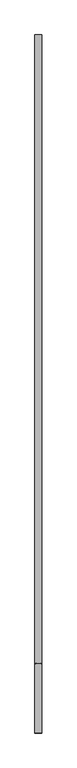
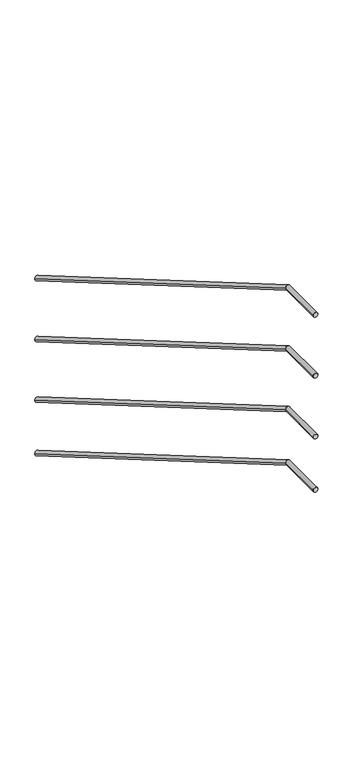
"""IFC4 building model written with IfcOpenShell, lengths in millimetres: railing geometry."""

from ifc_helpers import new_model, si_unit, frame, origin, place, context, project, spatial, circle_curve, ellipse_curve, source, transform, mapped, element, save
from ifc_brep_helpers import plane_surface, cylinder_surface, advanced_brep


def railing_4ce2e709(model_context):
    return source(origin(), model_context, "Body", "AdvancedBrep", [
        advanced_brep(
        [(-340.4, 15799.5208589, 8657.5963084), (-310.4, 15799.5208589, 8657.5963084), (-340.4, 13095.4656218, 10234.9618634), (-310.4, 13095.4656218, 10234.9618634), (-340.4, 12799.5208589, 10234.9618634), (-310.4, 12799.5208589, 10234.9618634)],
        [
            (0, 1, ellipse_curve(frame((-325.4, 15799.5208589, 8657.5963084), z_axis=(0.0, 1.0, 0.0), x_axis=(0.0, 0.0, -1.0)), 17.365555, 15.0)),
            (1, 0, ellipse_curve(frame((-325.4, 15799.5208589, 8657.5963084), z_axis=(0.0, 1.0, 0.0), x_axis=(0.0, 0.0, -1.0)), 17.365555, 15.0)),
            (0, 2),
            (2, 3, ellipse_curve(frame((-325.4, 13095.4656218, 10234.9618634), z_axis=(0.0, 0.965344213454049, -0.26097997921446664), x_axis=(0.0, -0.260979979214466, -0.9653442134540492)), 15.5384989, 15.0)),
            (3, 1),
            (3, 2, ellipse_curve(frame((-325.4, 13095.4656218, 10234.9618634), z_axis=(0.0, 0.965344213454049, -0.26097997921446664), x_axis=(0.0, -0.260979979214466, -0.9653442134540492)), 15.5384989, 15.0)),
            (4, 5, circle_curve(frame((-325.4, 12799.5208589, 10234.9618634), z_axis=(0.0, -1.0, 0.0), x_axis=(1.0, 0.0, 0.0)), 15.0)),
            (5, 4, circle_curve(frame((-325.4, 12799.5208589, 10234.9618634), z_axis=(0.0, -1.0, 0.0), x_axis=(1.0, 0.0, 0.0)), 15.0)),
            (2, 4),
            (5, 3),
        ],
        [
            plane_surface(frame((-325.4, 15799.5208589, 8674.9618634), z_axis=(0.0, 1.0, 0.0), x_axis=(0.0, 0.0, -1.0))),
            cylinder_surface(frame((-325.4, 15791.9627935, 8662.0051799), z_axis=(0.0, 0.8637789008984332, -0.5038710255240866), x_axis=(1.0, 0.0, 0.0)), 15.0),
            plane_surface(frame((-325.4, 12799.5208589, 10249.9618634), z_axis=(0.0, -1.0, 0.0), x_axis=(0.0, 0.0, -1.0))),
            cylinder_surface(frame((-325.4, 13099.5208589, 10234.9618634), z_axis=(0.0, 1.0, 0.0), x_axis=(1.0, 0.0, 0.0)), 15.0),
        ],
        [
            (0, [[1, 2]]),
            (1, [[-1, 3, 4, 5]]),
            (1, [[-2, -5, 6, -3]]),
            (2, [[7, 8]]),
            (3, [[-4, 9, -8, 10]]),
            (3, [[-6, -10, -7, -9]]),
        ],
    ),
        advanced_brep(
        [(-340.4, 15799.5208589, 7857.5963084), (-310.4, 15799.5208589, 7857.5963084), (-340.4, 13095.4656218, 9434.9618634), (-310.4, 13095.4656218, 9434.9618634), (-340.4, 12799.5208589, 9434.9618634), (-310.4, 12799.5208589, 9434.9618634)],
        [
            (0, 1, ellipse_curve(frame((-325.4, 15799.5208589, 7857.5963084), z_axis=(0.0, 1.0, 0.0), x_axis=(0.0, 0.0, -1.0)), 17.365555, 15.0)),
            (1, 0, ellipse_curve(frame((-325.4, 15799.5208589, 7857.5963084), z_axis=(0.0, 1.0, 0.0), x_axis=(0.0, 0.0, -1.0)), 17.365555, 15.0)),
            (0, 2),
            (2, 3, ellipse_curve(frame((-325.4, 13095.4656218, 9434.9618634), z_axis=(0.0, 0.965344213454049, -0.26097997921446664), x_axis=(0.0, -0.260979979214466, -0.9653442134540492)), 15.5384989, 15.0)),
            (3, 1),
            (3, 2, ellipse_curve(frame((-325.4, 13095.4656218, 9434.9618634), z_axis=(0.0, 0.965344213454049, -0.26097997921446664), x_axis=(0.0, -0.260979979214466, -0.9653442134540492)), 15.5384989, 15.0)),
            (4, 5, circle_curve(frame((-325.4, 12799.5208589, 9434.9618634), z_axis=(0.0, -1.0, 0.0), x_axis=(1.0, 0.0, 0.0)), 15.0)),
            (5, 4, circle_curve(frame((-325.4, 12799.5208589, 9434.9618634), z_axis=(0.0, -1.0, 0.0), x_axis=(1.0, 0.0, 0.0)), 15.0)),
            (2, 4),
            (5, 3),
        ],
        [
            plane_surface(frame((-325.4, 15799.5208589, 7874.9618634), z_axis=(0.0, 1.0, 0.0), x_axis=(0.0, 0.0, -1.0))),
            cylinder_surface(frame((-325.4, 15791.9627935, 7862.0051799), z_axis=(0.0, 0.8637789008984332, -0.5038710255240866), x_axis=(1.0, 0.0, 0.0)), 15.0),
            plane_surface(frame((-325.4, 12799.5208589, 9449.9618634), z_axis=(0.0, -1.0, 0.0), x_axis=(0.0, 0.0, -1.0))),
            cylinder_surface(frame((-325.4, 13099.5208589, 9434.9618634), z_axis=(0.0, 1.0, 0.0), x_axis=(1.0, 0.0, 0.0)), 15.0),
        ],
        [
            (0, [[1, 2]]),
            (1, [[-1, 3, 4, 5]]),
            (1, [[-2, -5, 6, -3]]),
            (2, [[7, 8]]),
            (3, [[-4, 9, -8, 10]]),
            (3, [[-6, -10, -7, -9]]),
        ],
    ),
        advanced_brep(
        [(-340.4, 15799.5208589, 8257.5963084), (-310.4, 15799.5208589, 8257.5963084), (-340.4, 13095.4656218, 9834.9618634), (-310.4, 13095.4656218, 9834.9618634), (-340.4, 12799.5208589, 9834.9618634), (-310.4, 12799.5208589, 9834.9618634)],
        [
            (0, 1, ellipse_curve(frame((-325.4, 15799.5208589, 8257.5963084), z_axis=(0.0, 1.0, 0.0), x_axis=(0.0, 0.0, -1.0)), 17.365555, 15.0)),
            (1, 0, ellipse_curve(frame((-325.4, 15799.5208589, 8257.5963084), z_axis=(0.0, 1.0, 0.0), x_axis=(0.0, 0.0, -1.0)), 17.365555, 15.0)),
            (0, 2),
            (2, 3, ellipse_curve(frame((-325.4, 13095.4656218, 9834.9618634), z_axis=(0.0, 0.965344213454049, -0.26097997921446664), x_axis=(0.0, -0.260979979214466, -0.9653442134540492)), 15.5384989, 15.0)),
            (3, 1),
            (3, 2, ellipse_curve(frame((-325.4, 13095.4656218, 9834.9618634), z_axis=(0.0, 0.965344213454049, -0.26097997921446664), x_axis=(0.0, -0.260979979214466, -0.9653442134540492)), 15.5384989, 15.0)),
            (4, 5, circle_curve(frame((-325.4, 12799.5208589, 9834.9618634), z_axis=(0.0, -1.0, 0.0), x_axis=(1.0, 0.0, 0.0)), 15.0)),
            (5, 4, circle_curve(frame((-325.4, 12799.5208589, 9834.9618634), z_axis=(0.0, -1.0, 0.0), x_axis=(1.0, 0.0, 0.0)), 15.0)),
            (2, 4),
            (5, 3),
        ],
        [
            plane_surface(frame((-325.4, 15799.5208589, 8274.9618634), z_axis=(0.0, 1.0, 0.0), x_axis=(0.0, 0.0, -1.0))),
            cylinder_surface(frame((-325.4, 15791.9627935, 8262.0051799), z_axis=(0.0, 0.8637789008984332, -0.5038710255240866), x_axis=(1.0, 0.0, 0.0)), 15.0),
            plane_surface(frame((-325.4, 12799.5208589, 9849.9618634), z_axis=(0.0, -1.0, 0.0), x_axis=(0.0, 0.0, -1.0))),
            cylinder_surface(frame((-325.4, 13099.5208589, 9834.9618634), z_axis=(0.0, 1.0, 0.0), x_axis=(1.0, 0.0, 0.0)), 15.0),
        ],
        [
            (0, [[1, 2]]),
            (1, [[-1, 3, 4, 5]]),
            (1, [[-2, -5, 6, -3]]),
            (2, [[7, 8]]),
            (3, [[-4, 9, -8, 10]]),
            (3, [[-6, -10, -7, -9]]),
        ],
    ),
        advanced_brep(
        [(-340.4, 15799.5208589, 7507.5963084), (-310.4, 15799.5208589, 7507.5963084), (-340.4, 13095.4656218, 9084.9618634), (-310.4, 13095.4656218, 9084.9618634), (-340.4, 12799.5208589, 9084.9618634), (-310.4, 12799.5208589, 9084.9618634)],
        [
            (0, 1, ellipse_curve(frame((-325.4, 15799.5208589, 7507.5963084), z_axis=(0.0, 1.0, 0.0), x_axis=(0.0, 0.0, -1.0)), 17.365555, 15.0)),
            (1, 0, ellipse_curve(frame((-325.4, 15799.5208589, 7507.5963084), z_axis=(0.0, 1.0, 0.0), x_axis=(0.0, 0.0, -1.0)), 17.365555, 15.0)),
            (0, 2),
            (2, 3, ellipse_curve(frame((-325.4, 13095.4656218, 9084.9618634), z_axis=(0.0, 0.965344213454049, -0.26097997921446664), x_axis=(0.0, -0.260979979214466, -0.9653442134540492)), 15.5384989, 15.0)),
            (3, 1),
            (3, 2, ellipse_curve(frame((-325.4, 13095.4656218, 9084.9618634), z_axis=(0.0, 0.965344213454049, -0.26097997921446664), x_axis=(0.0, -0.260979979214466, -0.9653442134540492)), 15.5384989, 15.0)),
            (4, 5, circle_curve(frame((-325.4, 12799.5208589, 9084.9618634), z_axis=(0.0, -1.0, 0.0), x_axis=(1.0, 0.0, 0.0)), 15.0)),
            (5, 4, circle_curve(frame((-325.4, 12799.5208589, 9084.9618634), z_axis=(0.0, -1.0, 0.0), x_axis=(1.0, 0.0, 0.0)), 15.0)),
            (2, 4),
            (5, 3),
        ],
        [
            plane_surface(frame((-325.4, 15799.5208589, 7524.9618634), z_axis=(0.0, 1.0, 0.0), x_axis=(0.0, 0.0, -1.0))),
            cylinder_surface(frame((-325.4, 15791.9627935, 7512.0051799), z_axis=(0.0, 0.8637789008984332, -0.5038710255240866), x_axis=(1.0, 0.0, 0.0)), 15.0),
            plane_surface(frame((-325.4, 12799.5208589, 9099.9618634), z_axis=(0.0, -1.0, 0.0), x_axis=(0.0, 0.0, -1.0))),
            cylinder_surface(frame((-325.4, 13099.5208589, 9084.9618634), z_axis=(0.0, 1.0, 0.0), x_axis=(1.0, 0.0, 0.0)), 15.0),
        ],
        [
            (0, [[1, 2]]),
            (1, [[-1, 3, 4, 5]]),
            (1, [[-2, -5, 6, -3]]),
            (2, [[7, 8]]),
            (3, [[-4, 9, -8, 10]]),
            (3, [[-6, -10, -7, -9]]),
        ],
    ),
    ])


if __name__ == "__main__":
    model = new_model("IFC4")
    model_context = context("Model", 3, world=origin())
    ifc_project = project(units=[si_unit("LENGTHUNIT", "METRE", prefix="MILLI")], contexts=[model_context])
    site = spatial("IfcSite", under=ifc_project)
    building = spatial("IfcBuilding", under=site)
    placement = place(None, origin())
    railing_shape = railing_4ce2e709(model_context)
    element("IfcRailing", 1, at=placement, inside=building, context=model_context, shape_type="MappedRepresentation", body=[
        mapped(railing_shape, transform((0.0, 0.0, 0.0), x_axis=(1.0, 0.0, 0.0), y_axis=(0.0, 1.0, 0.0), z_axis=(0.0, 0.0, 1.0))),
    ])
    save(model, "model.ifc")
